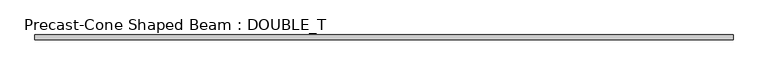
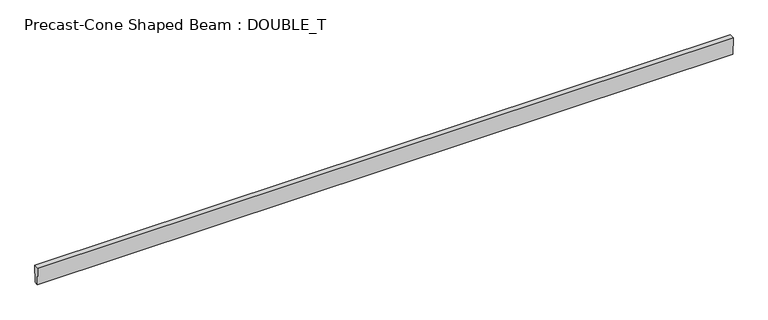
"""IFC4 building model written with IfcOpenShell, lengths in millimetres: beam geometry, Precast-Cone Shaped Beam : DOUBLE_T."""

import ifcopenshell
import ifcopenshell.guid

model = None  # the IFC model being written
_history = None  # IfcOwnerHistory: only IFC2X3 demands one
_inside = {}  # id of a spatial element -> (the spatial element, [elements in it])
_under = {}  # id of a project, library or spatial element -> (it, [spatial elements below it])
_declared = {}  # id of a project -> (the project, [libraries it declares])
_typed = {}  # id of a type object -> (the type object, [elements of that type])
_made_of = {}  # id of a material, layer set ... -> (it, [elements and type objects made of it])


def new_model(schema):
    """Start an empty IFC model of exactly this schema.

    Asked for "IFC4X3", IfcOpenShell would pick the latest addendum, in which some entities
    have other attributes; the version numbers below select the first issue.
    IFC2X3 requires an IfcOwnerHistory on every rooted entity: one is made here for all.
    """
    global model, _history
    if schema == "IFC4X3":
        model = ifcopenshell.file(schema_version=(4, 3, 0, 0))
    else:
        model = ifcopenshell.file(schema=schema)
    _inside.clear()
    _under.clear()
    _declared.clear()
    _typed.clear()
    _made_of.clear()
    _history = None
    if model.schema == "IFC2X3":
        org = make("IfcOrganization", Name="unknown")
        user = make(
            "IfcPersonAndOrganization",
            ThePerson=make("IfcPerson", FamilyName="unknown"),
            TheOrganization=org,
        )
        app = make(
            "IfcApplication",
            ApplicationDeveloper=org,
            Version="unknown",
            ApplicationFullName="unknown",
            ApplicationIdentifier="unknown",
        )
        _history = make(
            "IfcOwnerHistory",
            OwningUser=user,
            OwningApplication=app,
            ChangeAction="ADDED",
            CreationDate=0,
        )
    return model


def make(cls, **values):
    """One entity of the class cls with the attributes given. An attribute that is None is left unset."""
    return model.create_entity(
        cls, **{name: value for name, value in values.items() if value is not None}
    )


def rooted(cls, **values):
    """An entity with a GlobalId (a new one), such as an element, a storey or a relation."""
    return make(cls, GlobalId=ifcopenshell.guid.new(), OwnerHistory=_history, **values)


def si_unit(unit_type, name, prefix=None):
    """IfcSIUnit, for example si_unit("LENGTHUNIT", "METRE", prefix="MILLI")."""
    return make("IfcSIUnit", UnitType=unit_type, Prefix=prefix, Name=name)


def assignment(units):
    """IfcUnitAssignment: the units of a project."""
    return None if units is None else make("IfcUnitAssignment", Units=units)


def point(xyz):
    """IfcCartesianPoint."""
    return None if xyz is None else make("IfcCartesianPoint", Coordinates=xyz)


def direction(xyz):
    """IfcDirection."""
    return None if xyz is None else make("IfcDirection", DirectionRatios=xyz)


def frame(location, z_axis=None, x_axis=None):
    """IfcAxis2Placement3D, a coordinate frame: its origin and axes. An axis left out is left unset."""
    return make(
        "IfcAxis2Placement3D",
        Location=point(location),
        Axis=direction(z_axis),
        RefDirection=direction(x_axis),
    )


def origin():
    """The frame at (0, 0, 0) with its axes left unset."""
    return frame((0.0, 0.0, 0.0))


def place(relative_to, where):
    """IfcLocalPlacement: puts the frame where relative to a parent placement (None: the world)."""
    return make(
        "IfcLocalPlacement", PlacementRelTo=relative_to, RelativePlacement=where
    )


def context(
    kind, dimensions, precision=None, world=None, true_north=None, identifier=None
):
    """IfcGeometricRepresentationContext, for example the 3D "Model" context."""
    return make(
        "IfcGeometricRepresentationContext",
        ContextIdentifier=identifier,
        ContextType=kind,
        CoordinateSpaceDimension=dimensions,
        Precision=precision,
        WorldCoordinateSystem=world,
        TrueNorth=true_north,
    )


def project(units=None, contexts=None):
    """IfcProject with its units and contexts."""
    return rooted(
        "IfcProject",
        Name="project",
        RepresentationContexts=contexts,
        UnitsInContext=assignment(units),
    )


def spatial(cls, under=None, at=None, **own):
    """A site, building, storey or space (cls), placed at a placement, below another one or the project."""
    s = rooted(cls, ObjectPlacement=at, **own)
    if under is not None:
        _under.setdefault(under.id(), (under, []))[1].append(s)
    return s


def polyline(points):
    """IfcPolyline through the points."""
    return make("IfcPolyline", Points=[point(p) for p in points])


def outline(outer, holes=None, kind="AREA"):
    """IfcArbitraryClosedProfileDef: a profile drawn as a closed curve; with holes, ...WithVoids."""
    if holes is None:
        return make("IfcArbitraryClosedProfileDef", ProfileType=kind, OuterCurve=outer)
    return make(
        "IfcArbitraryProfileDefWithVoids",
        ProfileType=kind,
        OuterCurve=outer,
        InnerCurves=holes,
    )


def extrude(swept, where, along, depth):
    """IfcExtrudedAreaSolid: the profile swept, set in the frame where, extruded along a direction by depth."""
    return make(
        "IfcExtrudedAreaSolid",
        SweptArea=swept,
        Position=where,
        ExtrudedDirection=direction(along),
        Depth=depth,
    )


def shape(context_of_items, identifier, shape_type, items):
    """IfcShapeRepresentation: the items that make up one representation, for example the "Body"."""
    return make(
        "IfcShapeRepresentation",
        ContextOfItems=context_of_items,
        RepresentationIdentifier=identifier,
        RepresentationType=shape_type,
        Items=items,
    )


def source(mapping_origin, context_of_items, identifier, shape_type, items):
    """IfcRepresentationMap: a shape defined once, which mapped items show again and again."""
    return make(
        "IfcRepresentationMap",
        MappingOrigin=mapping_origin,
        MappedRepresentation=shape(context_of_items, identifier, shape_type, items),
    )


def transform(
    local_origin,
    x_axis=None,
    y_axis=None,
    z_axis=None,
    scale=None,
    scale2=None,
    scale3=None,
    uniform=True,
):
    """IfcCartesianTransformationOperator3D, or its non-uniform kind. x_axis, y_axis, z_axis: its Axis1, 2, 3."""
    if uniform:
        return make(
            "IfcCartesianTransformationOperator3D",
            Axis1=direction(x_axis),
            Axis2=direction(y_axis),
            LocalOrigin=point(local_origin),
            Scale=scale,
            Axis3=direction(z_axis),
        )
    return make(
        "IfcCartesianTransformationOperator3DnonUniform",
        Axis1=direction(x_axis),
        Axis2=direction(y_axis),
        LocalOrigin=point(local_origin),
        Scale=scale,
        Axis3=direction(z_axis),
        Scale2=scale2,
        Scale3=scale3,
    )


def mapped(mapping_source, mapping_target):
    """IfcMappedItem: shows the shape of a source again, moved by a transform."""
    return make(
        "IfcMappedItem", MappingSource=mapping_source, MappingTarget=mapping_target
    )


def made_of(thing, what):
    """Note that an element or type object is made of a material, layer set ...; save() writes the relation."""
    if what is not None:
        _made_of.setdefault(what.id(), (what, []))[1].append(thing)
    return thing


def element(
    cls,
    number,
    at=None,
    inside=None,
    cuts=None,
    type_object=None,
    material=None,
    context=None,
    identifier="Body",
    shape_type=None,
    held_by="IfcProductDefinitionShape",
    body=None,
    shapes=None,
    **own,
):
    """One element of the class cls, such as IfcWall. Its Tag is "e" and its number.

    at: its placement. inside: the storey or other place that contains it. cuts: it is an
    opening in that element (IfcRelVoidsElement). A single representation is given by context,
    identifier, shape_type and body (its items); several are given by shapes. held_by: the class
    of the entity that holds the representations. save() writes the other relations.
    """
    e = rooted(cls, Tag="e%d" % number, ObjectPlacement=at, **own)
    if body is not None:
        shapes = [shape(context, identifier, shape_type, body)]
    if shapes is not None:
        e.Representation = make(held_by, Representations=shapes)
    if inside is not None:
        _inside.setdefault(inside.id(), (inside, []))[1].append(e)
    if cuts is not None:
        rooted(
            "IfcRelVoidsElement", RelatingBuildingElement=cuts, RelatedOpeningElement=e
        )
    if type_object is not None:
        _typed.setdefault(type_object.id(), (type_object, []))[1].append(e)
    return made_of(e, material)


def aggregate(whole, parts):
    """IfcRelAggregates: a whole, such as a stair, and the parts it consists of."""
    return rooted("IfcRelAggregates", RelatingObject=whole, RelatedObjects=parts)


def save(model, path):
    """Write the relations noted so far, then the file.

    IfcRelAggregates (storeys below a building ...), IfcRelContainedInSpatialStructure (elements
    in a storey), IfcRelDefinesByType, IfcRelAssociatesMaterial and IfcRelDeclares: one each for
    every whole, place, type object, material and project.
    """
    for whole, parts in _under.values():
        aggregate(whole, parts)
    for where, things in _inside.values():
        rooted(
            "IfcRelContainedInSpatialStructure",
            RelatedElements=things,
            RelatingStructure=where,
        )
    for kind, things in _typed.values():
        rooted("IfcRelDefinesByType", RelatedObjects=things, RelatingType=kind)
    for what, things in _made_of.values():
        rooted("IfcRelAssociatesMaterial", RelatedObjects=things, RelatingMaterial=what)
    for by, libraries in _declared.values():
        rooted("IfcRelDeclares", RelatingContext=by, RelatedDefinitions=libraries)
    model.write(path)


def precast_cone_shaped_beam_double_t_d24bed89(model_context):
    return source(origin(), model_context, "Body", "SweptSolid", [
        extrude(outline(polyline([(-50.8, -228.6), (-63.5, 228.6), (63.5, 228.6), (50.8, -228.6), (-50.8, -228.6)])), frame((-8915.4, 0.0, 0.0), z_axis=(1.0, 0.0, 0.0), x_axis=(0.0, 1.0, 0.0)), (0.0, 0.0, 1.0), 17907.0),
    ])


if __name__ == "__main__":
    model = new_model("IFC4")
    model_context = context("Model", 3, world=origin())
    ifc_project = project(units=[si_unit("LENGTHUNIT", "METRE", prefix="MILLI")], contexts=[model_context])
    site = spatial("IfcSite", under=ifc_project)
    building = spatial("IfcBuilding", under=site)
    placement = place(None, origin())
    precast_cone_shaped_beam_double_t_shape = precast_cone_shaped_beam_double_t_d24bed89(model_context)
    element("IfcBeam", 1, ObjectType="Precast-Cone Shaped Beam : DOUBLE_T", at=placement, inside=building, context=model_context, shape_type="MappedRepresentation", body=[
        mapped(precast_cone_shaped_beam_double_t_shape, transform((0.0, 0.0, 0.0), x_axis=(1.0, 0.0, 0.0), y_axis=(0.0, 1.0, 0.0), z_axis=(0.0, 0.0, 1.0))),
    ])
    save(model, "model.ifc")

# Revit data of these elements
# Type "Precast-Cone Shaped Beam : DOUBLE_T"
#   Top Width = 0' - 5"
#   Tie Rod Weight [instance default] = 30
#   Tie Rod W [instance default] = 0.0660938 kip
#   Single Rebar Weight [instance default] = 50
#   Single Rebar W [instance default] = 0.110156 kip
#   Rebar Grids Weight [instance default] = 100
#   Rebar Grids W [instance default] = 0.220313 kip
#   Depth = 1' - 6"
#   Bottom Width = 0' - 4"
#   Length [instance default] = 5' - 0"
#   Structural Material [instance default] = Concrete, Precast
#   Assembly Code = ""
# Element 1 (IfcBeam, "Precast-Cone Shaped Beam : DOUBLE_T")
#   Length = 59' - 6"
#   Structural Material = Concrete - Precast Concrete - Normal Weight Concrete - 5 ksi
#   Materials on its faces: "Concrete - Precast Concrete - Normal Weight Concrete - 5 ksi"
# Materials
#   "Concrete, Precast": class "Concrete", colour RGB 198 187 187, transparency 0, Description = "Precast concrete", Cost = 0
#   "Concrete - Precast Concrete - Normal Weight Concrete - 5 ksi": class "Concrete", colour RGB 198 187 187, transparency 0, Cost = 0
